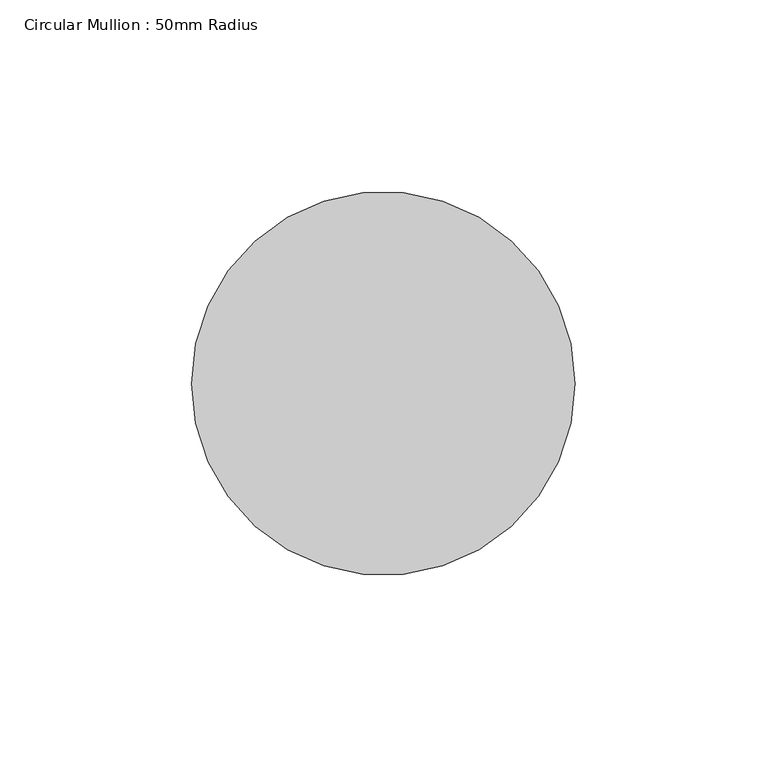
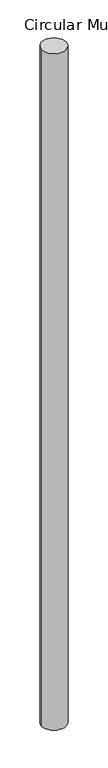
"""IFC4 building model written with IfcOpenShell, lengths in millimetres: member geometry, Circular Mullion : 50mm Radius."""

from ifc_helpers import new_model, si_unit, point, frame, frame_2d, origin, place, context, project, spatial, circle_curve, trimmed, segment, composite_curve, outline, extrude, source, transform, mapped, element, save


def circular_mullion_50mm_radius_d1c9c332(model_context):
    return source(origin(), model_context, "Body", "SweptSolid", [
        extrude(outline(composite_curve([segment(trimmed(circle_curve(frame_2d((-50.0, 0.0)), 50.0), [point((0.0, 0.0))], [point((-100.0, 0.0))], False, "CARTESIAN"), True, "CONTINUOUS"), segment(trimmed(circle_curve(frame_2d((-50.0, 0.0)), 50.0), [point((-100.0, 0.0))], [point((0.0, 0.0))], False, "CARTESIAN"), True, "CONTINUOUS")], self_intersect=False)), frame((0.0, 0.0, -2939.7028086), z_axis=(0.0, 0.0, 1.0), x_axis=(1.0, 0.0, 0.0)), (0.0, 0.0, 1.0), 2939.7028086),
    ])


if __name__ == "__main__":
    model = new_model("IFC4")
    model_context = context("Model", 3, world=origin())
    ifc_project = project(units=[si_unit("LENGTHUNIT", "METRE", prefix="MILLI")], contexts=[model_context])
    site = spatial("IfcSite", under=ifc_project)
    building = spatial("IfcBuilding", under=site)
    placement = place(None, origin())
    circular_mullion_50mm_radius_shape = circular_mullion_50mm_radius_d1c9c332(model_context)
    element("IfcMember", 1, ObjectType="Circular Mullion : 50mm Radius", at=placement, inside=building, context=model_context, shape_type="MappedRepresentation", body=[
        mapped(circular_mullion_50mm_radius_shape, transform((0.0, 0.0, 0.0), x_axis=(1.0, 0.0, 0.0), y_axis=(0.0, 1.0, 0.0), z_axis=(0.0, 0.0, 1.0))),
    ])
    save(model, "model.ifc")

# Revit data of these elements
# Type "Circular Mullion : 50mm Radius"
#   built-in parameter 1007350 = 0.164042 (stored number, unit not read)
# Element 1 (IfcMember, "Circular Mullion : 50mm Radius")
#   Materials on its faces: "Aluminium"
# Materials
#   "Aluminium": class "Metal", colour RGB 247 247 247, transparency 0, Description = "Aluminium 6061", Cost = 0
